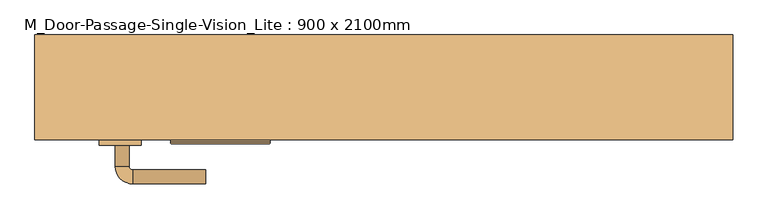
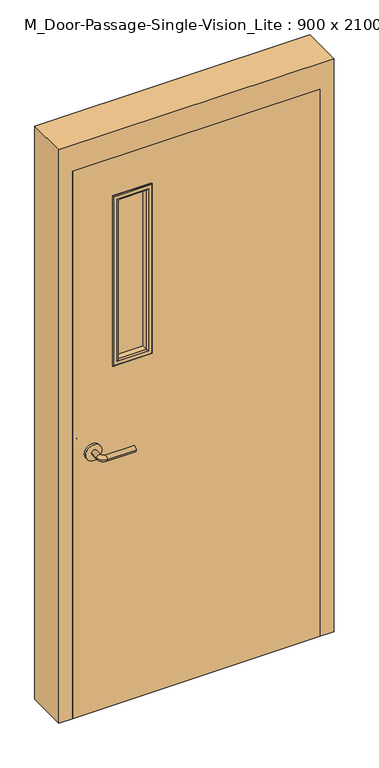
"""IFC4 building model written with IfcOpenShell, lengths in millimetres: door geometry, M_Door-Passage-Single-Vision_Lite : 900 x 2100mm."""

import ifcopenshell
import ifcopenshell.guid

model = None  # the IFC model being written
_history = None  # IfcOwnerHistory: only IFC2X3 demands one
_inside = {}  # id of a spatial element -> (the spatial element, [elements in it])
_under = {}  # id of a project, library or spatial element -> (it, [spatial elements below it])
_declared = {}  # id of a project -> (the project, [libraries it declares])
_typed = {}  # id of a type object -> (the type object, [elements of that type])
_made_of = {}  # id of a material, layer set ... -> (it, [elements and type objects made of it])


def new_model(schema):
    """Start an empty IFC model of exactly this schema.

    Asked for "IFC4X3", IfcOpenShell would pick the latest addendum, in which some entities
    have other attributes; the version numbers below select the first issue.
    IFC2X3 requires an IfcOwnerHistory on every rooted entity: one is made here for all.
    """
    global model, _history
    if schema == "IFC4X3":
        model = ifcopenshell.file(schema_version=(4, 3, 0, 0))
    else:
        model = ifcopenshell.file(schema=schema)
    _inside.clear()
    _under.clear()
    _declared.clear()
    _typed.clear()
    _made_of.clear()
    _history = None
    if model.schema == "IFC2X3":
        org = make("IfcOrganization", Name="unknown")
        user = make(
            "IfcPersonAndOrganization",
            ThePerson=make("IfcPerson", FamilyName="unknown"),
            TheOrganization=org,
        )
        app = make(
            "IfcApplication",
            ApplicationDeveloper=org,
            Version="unknown",
            ApplicationFullName="unknown",
            ApplicationIdentifier="unknown",
        )
        _history = make(
            "IfcOwnerHistory",
            OwningUser=user,
            OwningApplication=app,
            ChangeAction="ADDED",
            CreationDate=0,
        )
    return model


def make(cls, **values):
    """One entity of the class cls with the attributes given. An attribute that is None is left unset."""
    return model.create_entity(
        cls, **{name: value for name, value in values.items() if value is not None}
    )


def rooted(cls, **values):
    """An entity with a GlobalId (a new one), such as an element, a storey or a relation."""
    return make(cls, GlobalId=ifcopenshell.guid.new(), OwnerHistory=_history, **values)


def si_unit(unit_type, name, prefix=None):
    """IfcSIUnit, for example si_unit("LENGTHUNIT", "METRE", prefix="MILLI")."""
    return make("IfcSIUnit", UnitType=unit_type, Prefix=prefix, Name=name)


def assignment(units):
    """IfcUnitAssignment: the units of a project."""
    return None if units is None else make("IfcUnitAssignment", Units=units)


def point(xyz):
    """IfcCartesianPoint."""
    return None if xyz is None else make("IfcCartesianPoint", Coordinates=xyz)


def direction(xyz):
    """IfcDirection."""
    return None if xyz is None else make("IfcDirection", DirectionRatios=xyz)


def frame(location, z_axis=None, x_axis=None):
    """IfcAxis2Placement3D, a coordinate frame: its origin and axes. An axis left out is left unset."""
    return make(
        "IfcAxis2Placement3D",
        Location=point(location),
        Axis=direction(z_axis),
        RefDirection=direction(x_axis),
    )


def frame_2d(location, x_axis=None):
    """IfcAxis2Placement2D, a coordinate frame in the plane: its origin and x axis."""
    return make(
        "IfcAxis2Placement2D", Location=point(location), RefDirection=direction(x_axis)
    )


def origin():
    """The frame at (0, 0, 0) with its axes left unset."""
    return frame((0.0, 0.0, 0.0))


def place(relative_to, where):
    """IfcLocalPlacement: puts the frame where relative to a parent placement (None: the world)."""
    return make(
        "IfcLocalPlacement", PlacementRelTo=relative_to, RelativePlacement=where
    )


def context(
    kind, dimensions, precision=None, world=None, true_north=None, identifier=None
):
    """IfcGeometricRepresentationContext, for example the 3D "Model" context."""
    return make(
        "IfcGeometricRepresentationContext",
        ContextIdentifier=identifier,
        ContextType=kind,
        CoordinateSpaceDimension=dimensions,
        Precision=precision,
        WorldCoordinateSystem=world,
        TrueNorth=true_north,
    )


def project(units=None, contexts=None):
    """IfcProject with its units and contexts."""
    return rooted(
        "IfcProject",
        Name="project",
        RepresentationContexts=contexts,
        UnitsInContext=assignment(units),
    )


def spatial(cls, under=None, at=None, **own):
    """A site, building, storey or space (cls), placed at a placement, below another one or the project."""
    s = rooted(cls, ObjectPlacement=at, **own)
    if under is not None:
        _under.setdefault(under.id(), (under, []))[1].append(s)
    return s


def polyline(points):
    """IfcPolyline through the points."""
    return make("IfcPolyline", Points=[point(p) for p in points])


def circle_curve(where, radius):
    """IfcCircle in the frame where."""
    return make("IfcCircle", Position=where, Radius=radius)


def ellipse_curve(where, semi_axis1, semi_axis2):
    """IfcEllipse in the frame where."""
    return make(
        "IfcEllipse", Position=where, SemiAxis1=semi_axis1, SemiAxis2=semi_axis2
    )


def trimmed(basis, trim1, trim2, sense, master):
    """IfcTrimmedCurve: the piece of a basis curve between two trims."""
    return make(
        "IfcTrimmedCurve",
        BasisCurve=basis,
        Trim1=trim1,
        Trim2=trim2,
        SenseAgreement=sense,
        MasterRepresentation=master,
    )


def segment(curve, same_sense, transition):
    """IfcCompositeCurveSegment."""
    return make(
        "IfcCompositeCurveSegment",
        Transition=transition,
        SameSense=same_sense,
        ParentCurve=curve,
    )


def composite_curve(segments, self_intersect=None):
    """IfcCompositeCurve: segments joined end to end."""
    return make("IfcCompositeCurve", Segments=segments, SelfIntersect=self_intersect)


def outline(outer, holes=None, kind="AREA"):
    """IfcArbitraryClosedProfileDef: a profile drawn as a closed curve; with holes, ...WithVoids."""
    if holes is None:
        return make("IfcArbitraryClosedProfileDef", ProfileType=kind, OuterCurve=outer)
    return make(
        "IfcArbitraryProfileDefWithVoids",
        ProfileType=kind,
        OuterCurve=outer,
        InnerCurves=holes,
    )


def extrude(swept, where, along, depth):
    """IfcExtrudedAreaSolid: the profile swept, set in the frame where, extruded along a direction by depth."""
    return make(
        "IfcExtrudedAreaSolid",
        SweptArea=swept,
        Position=where,
        ExtrudedDirection=direction(along),
        Depth=depth,
    )


def faces_of(points, faces, orient=None, outer=None):
    """IfcFace entities. A face is a list of loops; a loop is a list of indices into points, from 0.

    orient and outer hold one flag for each loop. By default every Orientation is true, the
    first loop of a face is its IfcFaceOuterBound and the others are IfcFaceBound.
    """
    made = []
    for i, loops in enumerate(faces):
        bounds = []
        for j, loop in enumerate(loops):
            is_outer = j == 0 if outer is None else outer[i][j]
            bounds.append(
                make(
                    "IfcFaceOuterBound" if is_outer else "IfcFaceBound",
                    Bound=make("IfcPolyLoop", Polygon=[points[k] for k in loop]),
                    Orientation=True if orient is None else orient[i][j],
                )
            )
        made.append(make("IfcFace", Bounds=bounds))
    return made


def faceted_brep(points, faces, orient=None, outer=None, voids=None):
    """IfcFacetedBrep: a solid bounded by flat faces; with voids (closed shells), ...WithVoids."""
    shared = [point(p) for p in points]
    hull = make("IfcClosedShell", CfsFaces=faces_of(shared, faces, orient, outer))
    if voids is None:
        return make("IfcFacetedBrep", Outer=hull)
    return make(
        "IfcFacetedBrepWithVoids",
        Outer=hull,
        Voids=[
            make(cls, CfsFaces=faces_of(shared, fs, o, b)) for cls, fs, o, b in voids
        ],
    )


def shape(context_of_items, identifier, shape_type, items):
    """IfcShapeRepresentation: the items that make up one representation, for example the "Body"."""
    return make(
        "IfcShapeRepresentation",
        ContextOfItems=context_of_items,
        RepresentationIdentifier=identifier,
        RepresentationType=shape_type,
        Items=items,
    )


def source(mapping_origin, context_of_items, identifier, shape_type, items):
    """IfcRepresentationMap: a shape defined once, which mapped items show again and again."""
    return make(
        "IfcRepresentationMap",
        MappingOrigin=mapping_origin,
        MappedRepresentation=shape(context_of_items, identifier, shape_type, items),
    )


def transform(
    local_origin,
    x_axis=None,
    y_axis=None,
    z_axis=None,
    scale=None,
    scale2=None,
    scale3=None,
    uniform=True,
):
    """IfcCartesianTransformationOperator3D, or its non-uniform kind. x_axis, y_axis, z_axis: its Axis1, 2, 3."""
    if uniform:
        return make(
            "IfcCartesianTransformationOperator3D",
            Axis1=direction(x_axis),
            Axis2=direction(y_axis),
            LocalOrigin=point(local_origin),
            Scale=scale,
            Axis3=direction(z_axis),
        )
    return make(
        "IfcCartesianTransformationOperator3DnonUniform",
        Axis1=direction(x_axis),
        Axis2=direction(y_axis),
        LocalOrigin=point(local_origin),
        Scale=scale,
        Axis3=direction(z_axis),
        Scale2=scale2,
        Scale3=scale3,
    )


def mapped(mapping_source, mapping_target):
    """IfcMappedItem: shows the shape of a source again, moved by a transform."""
    return make(
        "IfcMappedItem", MappingSource=mapping_source, MappingTarget=mapping_target
    )


def made_of(thing, what):
    """Note that an element or type object is made of a material, layer set ...; save() writes the relation."""
    if what is not None:
        _made_of.setdefault(what.id(), (what, []))[1].append(thing)
    return thing


def element(
    cls,
    number,
    at=None,
    inside=None,
    cuts=None,
    type_object=None,
    material=None,
    context=None,
    identifier="Body",
    shape_type=None,
    held_by="IfcProductDefinitionShape",
    body=None,
    shapes=None,
    **own,
):
    """One element of the class cls, such as IfcWall. Its Tag is "e" and its number.

    at: its placement. inside: the storey or other place that contains it. cuts: it is an
    opening in that element (IfcRelVoidsElement). A single representation is given by context,
    identifier, shape_type and body (its items); several are given by shapes. held_by: the class
    of the entity that holds the representations. save() writes the other relations.
    """
    e = rooted(cls, Tag="e%d" % number, ObjectPlacement=at, **own)
    if body is not None:
        shapes = [shape(context, identifier, shape_type, body)]
    if shapes is not None:
        e.Representation = make(held_by, Representations=shapes)
    if inside is not None:
        _inside.setdefault(inside.id(), (inside, []))[1].append(e)
    if cuts is not None:
        rooted(
            "IfcRelVoidsElement", RelatingBuildingElement=cuts, RelatedOpeningElement=e
        )
    if type_object is not None:
        _typed.setdefault(type_object.id(), (type_object, []))[1].append(e)
    return made_of(e, material)


def aggregate(whole, parts):
    """IfcRelAggregates: a whole, such as a stair, and the parts it consists of."""
    return rooted("IfcRelAggregates", RelatingObject=whole, RelatedObjects=parts)


def save(model, path):
    """Write the relations noted so far, then the file.

    IfcRelAggregates (storeys below a building ...), IfcRelContainedInSpatialStructure (elements
    in a storey), IfcRelDefinesByType, IfcRelAssociatesMaterial and IfcRelDeclares: one each for
    every whole, place, type object, material and project.
    """
    for whole, parts in _under.values():
        aggregate(whole, parts)
    for where, things in _inside.values():
        rooted(
            "IfcRelContainedInSpatialStructure",
            RelatedElements=things,
            RelatingStructure=where,
        )
    for kind, things in _typed.values():
        rooted("IfcRelDefinesByType", RelatedObjects=things, RelatingType=kind)
    for what, things in _made_of.values():
        rooted("IfcRelAssociatesMaterial", RelatedObjects=things, RelatingMaterial=what)
    for by, libraries in _declared.values():
        rooted("IfcRelDeclares", RelatingContext=by, RelatedDefinitions=libraries)
    model.write(path)


def plane_surface(at):
    """IfcPlane: the flat surface through the origin of the frame at, square to its z axis."""
    return make("IfcPlane", Position=at)


def cylinder_surface(at, radius):
    """IfcCylindricalSurface: all points at the distance radius from the z axis of the frame at."""
    return make("IfcCylindricalSurface", Position=at, Radius=radius)


def revolved_surface(curve, axis_point, axis_direction):
    """IfcSurfaceOfRevolution: the curve turned about the line through axis_point along axis_direction."""
    return make(
        "IfcSurfaceOfRevolution",
        SweptCurve=make("IfcArbitraryOpenProfileDef", ProfileType="CURVE", Curve=curve),
        AxisPosition=make("IfcAxis1Placement", Location=point(axis_point), Axis=direction(axis_direction)),
    )


def advanced_brep(points, edges, surfaces, faces):
    """IfcAdvancedBrep: a solid bounded by faces that lie on surfaces and meet in shared edges.

    An edge is (start, end): straight between two places in points (the first is 0);
    or (start, end, curve); or (start, end, curve, False) where it runs against its curve.
    A face is (place in surfaces, loops), or (place, loops, False) where it looks against
    its surface's normal. A loop lists edges by number (the first is 1), with a minus sign
    where the edge is run from its end to its start. The first loop is the outer one.
    """
    corners = [point(p) for p in points]
    vertices = [make("IfcVertexPoint", VertexGeometry=c) for c in corners]
    made = []
    for start, end, *more in edges:
        made.append(
            make(
                "IfcEdgeCurve",
                EdgeStart=vertices[start],
                EdgeEnd=vertices[end],
                EdgeGeometry=more[0] if more else make("IfcPolyline", Points=[corners[start], corners[end]]),
                SameSense=more[1] if len(more) > 1 else True,
            )
        )
    hull = []
    for where, loops, *sense in faces:
        bounds = []
        for j, loop in enumerate(loops):
            ring = [make("IfcOrientedEdge", EdgeElement=made[abs(k) - 1], Orientation=k > 0) for k in loop]
            bounds.append(
                make(
                    "IfcFaceOuterBound" if j == 0 else "IfcFaceBound",
                    Bound=make("IfcEdgeLoop", EdgeList=ring),
                    Orientation=True,
                )
            )
        hull.append(make("IfcAdvancedFace", Bounds=bounds, FaceSurface=surfaces[where], SameSense=sense[0] if sense else True))
    return make("IfcAdvancedBrep", Outer=make("IfcClosedShell", CfsFaces=hull))


def m_door_passage_single_vision_lite_900_x_2100mm_db62f7dd(model_context):
    return source(origin(), model_context, "Body", "SolidModel", [
        advanced_brep(
        [(-384.990625, 9.15, 1000.0), (-364.990625, 9.15, 1000.0), (-384.990625, 39.15, 1000.0), (-364.990625, 39.15, 1000.0), (-359.990625, 44.15, 1000.0), (-359.990625, 64.15, 1000.0), (-254.990625, 64.15, 1000.0), (-254.990625, 44.15, 1000.0)],
        [
            (0, 1, circle_curve(frame((-374.990625, 9.15, 1000.0), z_axis=(0.0, -1.0, 0.0), x_axis=(1.0, 0.0, 0.0)), 10.0)),
            (1, 0, circle_curve(frame((-374.990625, 9.15, 1000.0), z_axis=(0.0, -1.0, 0.0), x_axis=(1.0, 0.0, 0.0)), 10.0)),
            (0, 2),
            (2, 3, circle_curve(frame((-374.990625, 39.15, 1000.0), z_axis=(0.0, -1.0, 0.0), x_axis=(1.0, 0.0, 0.0)), 10.0)),
            (3, 1),
            (3, 2, circle_curve(frame((-374.990625, 39.15, 1000.0), z_axis=(0.0, -1.0, 0.0), x_axis=(1.0, 0.0, 0.0)), 10.0)),
            (4, 3, circle_curve(frame((-359.990625, 39.15, 1000.0), z_axis=(0.0, 0.0, 1.0), x_axis=(-1.0, 0.0, 0.0)), 5.0)),
            (2, 5, circle_curve(frame((-359.990625, 39.15, 1000.0), z_axis=(0.0, 0.0, -1.0), x_axis=(-1.0, 0.0, 0.0)), 25.0)),
            (5, 4, circle_curve(frame((-359.990625, 54.15, 1000.0), z_axis=(-1.0, 0.0, 0.0), x_axis=(0.0, -1.0, 0.0)), 10.0)),
            (4, 5, circle_curve(frame((-359.990625, 54.15, 1000.0), z_axis=(-1.0, 0.0, 0.0), x_axis=(0.0, -1.0, 0.0)), 10.0)),
            (6, 7, circle_curve(frame((-254.990625, 54.15, 1000.0), z_axis=(1.0, 0.0, 0.0), x_axis=(0.0, -1.0, 0.0)), 10.0)),
            (7, 6, circle_curve(frame((-254.990625, 54.15, 1000.0), z_axis=(1.0, 0.0, 0.0), x_axis=(0.0, -1.0, 0.0)), 10.0)),
            (5, 6),
            (7, 4),
        ],
        [
            plane_surface(frame((-374.990625, 9.15, 1000.0), z_axis=(0.0, -1.0, 0.0), x_axis=(0.0, 0.0, 1.0))),
            cylinder_surface(frame((-374.990625, 9.15, 1000.0), z_axis=(0.0, -1.0, 0.0), x_axis=(1.0, 0.0, 0.0)), 10.0),
            revolved_surface(trimmed(ellipse_curve(frame((-374.990625, 39.15, 1000.0), z_axis=(0.0, -1.0, 0.0), x_axis=(1.0, 0.0, 0.0)), 10.0, 10.0), [point((-384.990625, 39.15, 1000.0))], [point((-364.990625, 39.15, 1000.0))], True, "CARTESIAN"), (-359.990625, 39.15, 1000.0), (0.0, 0.0, -1.0)),
            revolved_surface(trimmed(ellipse_curve(frame((-374.990625, 39.15, 1000.0), z_axis=(0.0, -1.0, 0.0), x_axis=(1.0, 0.0, 0.0)), 10.0, 10.0), [point((-364.990625, 39.15, 1000.0))], [point((-384.990625, 39.15, 1000.0))], True, "CARTESIAN"), (-359.990625, 39.15, 1000.0), (0.0, 0.0, -1.0)),
            plane_surface(frame((-254.990625, 54.15, 1000.0), z_axis=(1.0, 0.0, 0.0), x_axis=(0.0, 0.0, 1.0))),
            cylinder_surface(frame((-359.990625, 54.15, 1000.0), z_axis=(-1.0, 0.0, 0.0), x_axis=(0.0, -1.0, 0.0)), 10.0),
        ],
        [
            (0, [[1, 2]]),
            (1, [[-1, 3, 4, 5]]),
            (1, [[-2, -5, 6, -3]]),
            (2, [[7, -4, 8, 9]]),
            (3, [[-8, -6, -7, 10]]),
            (4, [[11, 12]]),
            (5, [[-9, 13, -12, 14]]),
            (5, [[-10, -14, -11, -13]]),
        ],
    ),
        extrude(outline(composite_curve([segment(trimmed(circle_curve(frame_2d((1000.0, -377.490625)), 30.0), [point((1000.0, -407.490625))], [point((1000.0, -347.490625))], False, "CARTESIAN"), True, "CONTINUOUS"), segment(trimmed(circle_curve(frame_2d((1000.0, -377.490625)), 30.0), [point((1000.0, -347.490625))], [point((1000.0, -407.490625))], False, "CARTESIAN"), True, "CONTINUOUS")], self_intersect=False)), frame((0.0, 1.15, 0.0), z_axis=(0.0, 1.0, 0.0), x_axis=(0.0, 0.0, 1.0)), (0.0, 0.0, 1.0), 8.0),
        advanced_brep(
        [(-384.990625, -51.85, 1000.0), (-364.990625, -51.85, 1000.0), (-364.990625, -81.85, 1000.0), (-384.990625, -81.85, 1000.0), (-359.990625, -86.85, 1000.0), (-359.990625, -106.85, 1000.0), (-254.990625, -106.85, 1000.0), (-254.990625, -86.85, 1000.0)],
        [
            (0, 1, circle_curve(frame((-374.990625, -51.85, 1000.0), z_axis=(0.0, 1.0, 0.0), x_axis=(1.0, 0.0, 0.0)), 10.0)),
            (1, 0, circle_curve(frame((-374.990625, -51.85, 1000.0), z_axis=(0.0, 1.0, 0.0), x_axis=(1.0, 0.0, 0.0)), 10.0)),
            (1, 2),
            (2, 3, circle_curve(frame((-374.990625, -81.85, 1000.0), z_axis=(0.0, 1.0, 0.0), x_axis=(1.0, 0.0, 0.0)), 10.0)),
            (3, 0),
            (3, 2, circle_curve(frame((-374.990625, -81.85, 1000.0), z_axis=(0.0, 1.0, 0.0), x_axis=(1.0, 0.0, 0.0)), 10.0)),
            (4, 5, circle_curve(frame((-359.990625, -96.85, 1000.0), z_axis=(-1.0, 0.0, 0.0), x_axis=(0.0, 1.0, 0.0)), 10.0)),
            (5, 3, circle_curve(frame((-359.990625, -81.85, 1000.0), z_axis=(0.0, 0.0, -1.0), x_axis=(-1.0, 0.0, 0.0)), 25.0)),
            (2, 4, circle_curve(frame((-359.990625, -81.85, 1000.0), z_axis=(0.0, 0.0, 1.0), x_axis=(-1.0, 0.0, 0.0)), 5.0)),
            (5, 4, circle_curve(frame((-359.990625, -96.85, 1000.0), z_axis=(-1.0, 0.0, 0.0), x_axis=(0.0, 1.0, 0.0)), 10.0)),
            (6, 7, circle_curve(frame((-254.990625, -96.85, 1000.0), z_axis=(1.0, 0.0, 0.0), x_axis=(0.0, 1.0, 0.0)), 10.0)),
            (7, 6, circle_curve(frame((-254.990625, -96.85, 1000.0), z_axis=(1.0, 0.0, 0.0), x_axis=(0.0, 1.0, 0.0)), 10.0)),
            (4, 7),
            (6, 5),
        ],
        [
            plane_surface(frame((-374.990625, -51.85, 1000.0), z_axis=(0.0, 1.0, 0.0), x_axis=(0.0, 0.0, 1.0))),
            cylinder_surface(frame((-374.990625, -51.85, 1000.0), z_axis=(0.0, 1.0, 0.0), x_axis=(1.0, 0.0, 0.0)), 10.0),
            revolved_surface(trimmed(ellipse_curve(frame((-374.990625, -81.85, 1000.0), z_axis=(0.0, -1.0, 0.0), x_axis=(1.0, 0.0, 0.0)), 10.0, 10.0), [point((-384.990625, -81.85, 1000.0))], [point((-364.990625, -81.85, 1000.0))], True, "CARTESIAN"), (-359.990625, -81.85, 1000.0), (0.0, 0.0, -1.0)),
            revolved_surface(trimmed(ellipse_curve(frame((-374.990625, -81.85, 1000.0), z_axis=(0.0, -1.0, 0.0), x_axis=(1.0, 0.0, 0.0)), 10.0, 10.0), [point((-364.990625, -81.85, 1000.0))], [point((-384.990625, -81.85, 1000.0))], True, "CARTESIAN"), (-359.990625, -81.85, 1000.0), (0.0, 0.0, -1.0)),
            plane_surface(frame((-254.990625, -96.85, 1000.0), z_axis=(1.0, 0.0, 0.0), x_axis=(0.0, 0.0, 1.0))),
            cylinder_surface(frame((-359.990625, -96.85, 1000.0), z_axis=(-1.0, 0.0, 0.0), x_axis=(0.0, 1.0, 0.0)), 10.0),
        ],
        [
            (0, [[1, 2]]),
            (1, [[3, 4, 5, -2]]),
            (1, [[-5, 6, -3, -1]]),
            (2, [[7, 8, -4, 9]]),
            (3, [[10, -9, -6, -8]]),
            (4, [[11, 12]]),
            (5, [[13, -11, 14, -7]]),
            (5, [[-14, -12, -13, -10]]),
        ],
    ),
        extrude(outline(composite_curve([segment(trimmed(circle_curve(frame_2d((1000.0, -377.490625)), 30.0), [point((1000.0, -407.490625))], [point((1000.0, -347.490625))], False, "CARTESIAN"), True, "CONTINUOUS"), segment(trimmed(circle_curve(frame_2d((1000.0, -377.490625)), 30.0), [point((1000.0, -347.490625))], [point((1000.0, -407.490625))], False, "CARTESIAN"), True, "CONTINUOUS")], self_intersect=False)), frame((0.0, -51.85, 0.0), z_axis=(0.0, 1.0, 0.0), x_axis=(0.0, 0.0, 1.0)), (0.0, 0.0, 1.0), 8.0),
        extrude(outline(polyline([(2100.0, -450.0), (0.0, -450.0), (0.0, 450.0), (2100.0, 450.0), (2100.0, -450.0)]), holes=[polyline([(1947.6, -297.6), (1947.6, -170.6), (1312.6, -170.6), (1312.6, -297.6), (1947.6, -297.6)])]), frame((0.0, -43.85, 0.0), z_axis=(0.0, 1.0, 0.0), x_axis=(0.0, 0.0, 1.0)), (0.0, 0.0, 1.0), 45.0),
        faceted_brep([(450.0, 5.9125, 0.0), (434.125, 5.9125, 0.0), (434.125, 56.9375, 0.0), (450.0, 56.9375, 0.0), (450.0, 106.15, 0.0), (500.0, 106.15, 0.0), (500.0, -43.85, 0.0), (450.0, -43.85, 0.0), (450.0, -43.85, 2100.0), (450.0, 5.9125, 2100.0), (500.0, -43.85, 2200.0), (-500.0, -43.85, 2200.0), (-500.0, -43.85, 0.0), (-450.0, -43.85, 0.0), (-450.0, -43.85, 2100.0), (500.0, 106.15, 2200.0), (450.0, 106.15, 2100.0), (-450.0, 106.15, 2100.0), (-450.0, 106.15, 0.0), (-500.0, 106.15, 0.0), (-500.0, 106.15, 2200.0), (450.0, 56.9375, 2100.0), (434.125, 56.9375, 2084.125), (-434.125, 56.9375, 2084.125), (-434.125, 56.9375, 0.0), (-450.0, 56.9375, 0.0), (-450.0, 56.9375, 2100.0), (434.125, 5.9125, 2084.125), (-450.0, 5.9125, 2100.0), (-450.0, 5.9125, 0.0), (-434.125, 5.9125, 0.0), (-434.125, 5.9125, 2084.125)], [[[0, 1, 2, 3, 4, 5, 6, 7]], [[7, 8, 9, 0]], [[6, 10, 11, 12, 13, 14, 8, 7]], [[5, 15, 10, 6]], [[4, 16, 17, 18, 19, 20, 15, 5]], [[3, 21, 16, 4]], [[2, 22, 23, 24, 25, 26, 21, 3]], [[1, 27, 22, 2]], [[0, 9, 28, 29, 30, 31, 27, 1]], [[8, 14, 28, 9]], [[16, 21, 26, 17]], [[22, 27, 31, 23]], [[12, 19, 18, 25, 24, 30, 29, 13]], [[13, 29, 28, 14]], [[11, 20, 19, 12]], [[17, 26, 25, 18]], [[23, 31, 30, 24]], [[15, 20, 11, 10]]]),
        extrude(outline(polyline([(-170.6, -18.85), (-170.6, -23.85), (-297.6, -23.85), (-297.6, -18.85), (-170.6, -18.85)])), frame((0.0, 0.0, 1312.6), z_axis=(0.0, 0.0, 1.0), x_axis=(1.0, 0.0, 0.0)), (0.0, 0.0, 1.0), 635.0),
        advanced_brep(
        [(-297.6, -23.85, 1947.6), (-297.6, -23.85, 1312.6), (-297.6, -43.85, 1312.6), (-297.6, -43.85, 1947.6), (-285.6, -44.85, 1935.6), (-285.6, -44.85, 1324.6), (-285.6, -23.85, 1324.6), (-285.6, -23.85, 1935.6), (-290.6, -49.85, 1940.6), (-290.6, -49.85, 1319.6), (-305.6, -47.85, 1955.6), (-305.6, -47.85, 1304.6), (-303.6, -49.85, 1306.6), (-303.6, -49.85, 1953.6), (-305.6, -43.85, 1955.6), (-305.6, -43.85, 1304.6), (-170.6, -23.85, 1312.6), (-170.6, -43.85, 1312.6), (-182.6, -44.85, 1324.6), (-182.6, -23.85, 1324.6), (-177.6, -49.85, 1319.6), (-162.6, -47.85, 1304.6), (-164.6, -49.85, 1306.6), (-162.6, -43.85, 1304.6), (-170.6, -23.85, 1947.6), (-170.6, -43.85, 1947.6), (-182.6, -44.85, 1935.6), (-182.6, -23.85, 1935.6), (-177.6, -49.85, 1940.6), (-162.6, -47.85, 1955.6), (-164.6, -49.85, 1953.6), (-162.6, -43.85, 1955.6)],
        [
            (0, 1),
            (1, 2),
            (2, 3),
            (3, 0),
            (4, 5),
            (5, 6),
            (6, 7),
            (7, 4),
            (8, 9),
            (9, 5, ellipse_curve(frame((-290.6, -44.85, 1319.6), z_axis=(-0.7071067811865475, 0.0, 0.7071067811865475), x_axis=(0.7071067811865474, 0.0, 0.7071067811865476)), 7.0710678, 5.0)),
            (4, 8, ellipse_curve(frame((-290.6, -44.85, 1940.6), z_axis=(-0.7071067811865475, 0.0, -0.7071067811865475), x_axis=(-0.7071067811865474, 0.0, 0.7071067811865476)), 7.0710678, 5.0)),
            (10, 11),
            (11, 12, ellipse_curve(frame((-303.6, -47.85, 1306.6), z_axis=(-0.7071067811865475, 0.0, 0.7071067811865475), x_axis=(0.7071067811865474, 0.0, 0.7071067811865476)), 2.8284271, 2.0)),
            (12, 13),
            (13, 10, ellipse_curve(frame((-303.6, -47.85, 1953.6), z_axis=(-0.7071067811865475, 0.0, -0.7071067811865475), x_axis=(-0.7071067811865474, 0.0, 0.7071067811865476)), 2.8284271, 2.0)),
            (14, 15),
            (15, 11),
            (10, 14),
            (1, 16),
            (16, 17),
            (17, 2),
            (5, 18),
            (18, 19),
            (19, 6),
            (9, 20),
            (20, 18, ellipse_curve(frame((-177.6, -44.85, 1319.6), z_axis=(-0.7071067811865475, 0.0, -0.7071067811865475), x_axis=(-0.7071067811865476, 0.0, 0.7071067811865474)), 7.0710678, 5.0)),
            (11, 21),
            (21, 22, ellipse_curve(frame((-164.6, -47.85, 1306.6), z_axis=(-0.7071067811865475, 0.0, -0.7071067811865475), x_axis=(-0.7071067811865476, 0.0, 0.7071067811865474)), 2.8284271, 2.0)),
            (22, 12),
            (15, 23),
            (23, 21),
            (16, 24),
            (24, 25),
            (25, 17),
            (18, 26),
            (26, 27),
            (27, 19),
            (20, 28),
            (28, 26, ellipse_curve(frame((-177.6, -44.85, 1940.6), z_axis=(0.7071067811865475, 0.0, -0.7071067811865475), x_axis=(-0.7071067811865474, 0.0, -0.7071067811865476)), 7.0710678, 5.0)),
            (21, 29),
            (29, 30, ellipse_curve(frame((-164.6, -47.85, 1953.6), z_axis=(0.7071067811865475, 0.0, -0.7071067811865475), x_axis=(-0.7071067811865474, 0.0, -0.7071067811865476)), 2.8284271, 2.0)),
            (30, 22),
            (23, 31),
            (31, 29),
            (14, 31),
            (25, 3),
            (24, 0),
            (27, 7),
            (26, 4),
            (28, 8),
            (30, 13),
            (29, 10),
        ],
        [
            plane_surface(frame((-297.6, -43.85, 1947.6), z_axis=(-1.0, 0.0, 0.0), x_axis=(0.0, 0.0, -1.0))),
            plane_surface(frame((-285.6, -23.85, 1935.6), z_axis=(1.0, 0.0, 0.0), x_axis=(0.0, 0.0, -1.0))),
            cylinder_surface(frame((-290.6, -44.85, 1947.6), z_axis=(0.0, 0.0, 1.0), x_axis=(-1.0, 0.0, 0.0)), 5.0),
            cylinder_surface(frame((-303.6, -47.85, 1947.6), z_axis=(0.0, 0.0, 1.0), x_axis=(-1.0, 0.0, 0.0)), 2.0),
            plane_surface(frame((-305.6, -47.85, 1955.6), z_axis=(-1.0, 0.0, 0.0), x_axis=(0.0, 0.0, -1.0))),
            plane_surface(frame((-297.6, -43.85, 1312.6), z_axis=(0.0, 0.0, -1.0), x_axis=(1.0, 0.0, 0.0))),
            plane_surface(frame((-285.6, -23.85, 1324.6), z_axis=(0.0, 0.0, 1.0), x_axis=(1.0, 0.0, 0.0))),
            cylinder_surface(frame((-297.6, -44.85, 1319.6), z_axis=(-1.0, 0.0, 0.0), x_axis=(0.0, 0.0, -1.0)), 5.0),
            cylinder_surface(frame((-297.6, -47.85, 1306.6), z_axis=(-1.0, 0.0, 0.0), x_axis=(0.0, 0.0, -1.0)), 2.0),
            plane_surface(frame((-305.6, -47.85, 1304.6), z_axis=(0.0, 0.0, -1.0), x_axis=(1.0, 0.0, 0.0))),
            plane_surface(frame((-170.6, -43.85, 1312.6), z_axis=(1.0, 0.0, 0.0), x_axis=(0.0, 0.0, 1.0))),
            plane_surface(frame((-182.6, -23.85, 1324.6), z_axis=(-1.0, 0.0, 0.0), x_axis=(0.0, 0.0, 1.0))),
            cylinder_surface(frame((-177.6, -44.85, 1312.6), z_axis=(0.0, 0.0, -1.0), x_axis=(1.0, 0.0, 0.0)), 5.0),
            cylinder_surface(frame((-164.6, -47.85, 1312.6), z_axis=(0.0, 0.0, -1.0), x_axis=(1.0, 0.0, 0.0)), 2.0),
            plane_surface(frame((-162.6, -47.85, 1304.6), z_axis=(1.0, 0.0, 0.0), x_axis=(0.0, 0.0, 1.0))),
            plane_surface(frame((-162.6, -43.85, 1955.6), z_axis=(0.0, 1.0, 0.0), x_axis=(-1.0, 0.0, 0.0))),
            plane_surface(frame((-170.6, -43.85, 1947.6), z_axis=(0.0, 0.0, 1.0), x_axis=(-1.0, 0.0, 0.0))),
            plane_surface(frame((-170.6, -23.85, 1947.6), z_axis=(0.0, 1.0, 0.0), x_axis=(-1.0, 0.0, 0.0))),
            plane_surface(frame((-182.6, -23.85, 1935.6), z_axis=(0.0, 0.0, -1.0), x_axis=(-1.0, 0.0, 0.0))),
            cylinder_surface(frame((-170.6, -44.85, 1940.6), z_axis=(1.0, 0.0, 0.0), x_axis=(0.0, 0.0, 1.0)), 5.0),
            plane_surface(frame((-177.6, -49.85, 1940.6), z_axis=(0.0, -1.0, 0.0), x_axis=(-1.0, 0.0, 0.0))),
            cylinder_surface(frame((-170.6, -47.85, 1953.6), z_axis=(1.0, 0.0, 0.0), x_axis=(0.0, 0.0, 1.0)), 2.0),
            plane_surface(frame((-162.6, -47.85, 1955.6), z_axis=(0.0, 0.0, 1.0), x_axis=(-1.0, 0.0, 0.0))),
        ],
        [
            (0, [[1, 2, 3, 4]]),
            (1, [[5, 6, 7, 8]]),
            (2, [[9, 10, -5, 11]]),
            (3, [[12, 13, 14, 15]]),
            (4, [[16, 17, -12, 18]]),
            (5, [[19, 20, 21, -2]]),
            (6, [[22, 23, 24, -6]]),
            (7, [[25, 26, -22, -10]]),
            (8, [[27, 28, 29, -13]]),
            (9, [[30, 31, -27, -17]]),
            (10, [[32, 33, 34, -20]]),
            (11, [[35, 36, 37, -23]]),
            (12, [[38, 39, -35, -26]]),
            (13, [[40, 41, 42, -28]]),
            (14, [[43, 44, -40, -31]]),
            (15, [[-16, 45, -43, -30], [-3, -21, -34, 46]]),
            (16, [[47, -4, -46, -33]]),
            (17, [[-1, -47, -32, -19], [-7, -24, -37, 48]]),
            (18, [[49, -8, -48, -36]]),
            (19, [[50, -11, -49, -39]]),
            (20, [[-14, -29, -42, 51], [-9, -50, -38, -25]]),
            (21, [[52, -15, -51, -41]]),
            (22, [[-45, -18, -52, -44]]),
        ],
    ),
        advanced_brep(
        [(-297.6, -18.85, 1312.6), (-297.6, -18.85, 1947.6), (-297.6, 1.15, 1947.6), (-297.6, 1.15, 1312.6), (-285.6, 2.15, 1324.6), (-285.6, 2.15, 1935.6), (-285.6, -18.85, 1935.6), (-285.6, -18.85, 1324.6), (-290.6, 7.15, 1319.6), (-290.6, 7.15, 1940.6), (-305.6, 5.15, 1304.6), (-305.6, 5.15, 1955.6), (-303.6, 7.15, 1953.6), (-303.6, 7.15, 1306.6), (-305.6, 1.15, 1304.6), (-305.6, 1.15, 1955.6), (-170.6, -18.85, 1947.6), (-170.6, 1.15, 1947.6), (-182.6, 2.15, 1935.6), (-182.6, -18.85, 1935.6), (-177.6, 7.15, 1940.6), (-162.6, 5.15, 1955.6), (-164.6, 7.15, 1953.6), (-162.6, 1.15, 1955.6), (-170.6, -18.85, 1312.6), (-170.6, 1.15, 1312.6), (-182.6, 2.15, 1324.6), (-182.6, -18.85, 1324.6), (-177.6, 7.15, 1319.6), (-162.6, 5.15, 1304.6), (-164.6, 7.15, 1306.6), (-162.6, 1.15, 1304.6)],
        [
            (0, 1),
            (1, 2),
            (2, 3),
            (3, 0),
            (4, 5),
            (5, 6),
            (6, 7),
            (7, 4),
            (8, 9),
            (9, 5, ellipse_curve(frame((-290.6, 2.15, 1940.6), z_axis=(-0.7071067811865475, 0.0, -0.7071067811865475), x_axis=(0.7071067811865474, 0.0, -0.7071067811865476)), 7.0710678, 5.0)),
            (4, 8, ellipse_curve(frame((-290.6, 2.15, 1319.6), z_axis=(-0.7071067811865475, 0.0, 0.7071067811865475), x_axis=(-0.7071067811865474, 0.0, -0.7071067811865476)), 7.0710678, 5.0)),
            (10, 11),
            (11, 12, ellipse_curve(frame((-303.6, 5.15, 1953.6), z_axis=(-0.7071067811865475, 0.0, -0.7071067811865475), x_axis=(0.7071067811865474, 0.0, -0.7071067811865476)), 2.8284271, 2.0)),
            (12, 13),
            (13, 10, ellipse_curve(frame((-303.6, 5.15, 1306.6), z_axis=(-0.7071067811865475, 0.0, 0.7071067811865475), x_axis=(-0.7071067811865474, 0.0, -0.7071067811865476)), 2.8284271, 2.0)),
            (14, 15),
            (15, 11),
            (10, 14),
            (1, 16),
            (16, 17),
            (17, 2),
            (5, 18),
            (18, 19),
            (19, 6),
            (9, 20),
            (20, 18, ellipse_curve(frame((-177.6, 2.15, 1940.6), z_axis=(-0.7071067811865475, 0.0, 0.7071067811865475), x_axis=(-0.7071067811865476, 0.0, -0.7071067811865474)), 7.0710678, 5.0)),
            (11, 21),
            (21, 22, ellipse_curve(frame((-164.6, 5.15, 1953.6), z_axis=(-0.7071067811865475, 0.0, 0.7071067811865475), x_axis=(-0.7071067811865476, 0.0, -0.7071067811865474)), 2.8284271, 2.0)),
            (22, 12),
            (15, 23),
            (23, 21),
            (16, 24),
            (24, 25),
            (25, 17),
            (18, 26),
            (26, 27),
            (27, 19),
            (20, 28),
            (28, 26, ellipse_curve(frame((-177.6, 2.15, 1319.6), z_axis=(0.7071067811865475, 0.0, 0.7071067811865475), x_axis=(-0.7071067811865474, 0.0, 0.7071067811865476)), 7.0710678, 5.0)),
            (21, 29),
            (29, 30, ellipse_curve(frame((-164.6, 5.15, 1306.6), z_axis=(0.7071067811865475, 0.0, 0.7071067811865475), x_axis=(-0.7071067811865474, 0.0, 0.7071067811865476)), 2.8284271, 2.0)),
            (30, 22),
            (23, 31),
            (31, 29),
            (14, 31),
            (25, 3),
            (24, 0),
            (27, 7),
            (26, 4),
            (28, 8),
            (30, 13),
            (29, 10),
        ],
        [
            plane_surface(frame((-297.6, 1.15, 1312.6), z_axis=(-1.0, 0.0, 0.0), x_axis=(0.0, 0.0, 1.0))),
            plane_surface(frame((-285.6, -18.85, 1324.6), z_axis=(1.0, 0.0, 0.0), x_axis=(0.0, 0.0, 1.0))),
            cylinder_surface(frame((-290.6, 2.15, 1312.6), z_axis=(0.0, 0.0, -1.0), x_axis=(-1.0, 0.0, 0.0)), 5.0),
            cylinder_surface(frame((-303.6, 5.15, 1312.6), z_axis=(0.0, 0.0, -1.0), x_axis=(-1.0, 0.0, 0.0)), 2.0),
            plane_surface(frame((-305.6, 5.15, 1304.6), z_axis=(-1.0, 0.0, 0.0), x_axis=(0.0, 0.0, 1.0))),
            plane_surface(frame((-297.6, 1.15, 1947.6), z_axis=(0.0, 0.0, 1.0), x_axis=(1.0, 0.0, 0.0))),
            plane_surface(frame((-285.6, -18.85, 1935.6), z_axis=(0.0, 0.0, -1.0), x_axis=(1.0, 0.0, 0.0))),
            cylinder_surface(frame((-297.6, 2.15, 1940.6), z_axis=(-1.0, 0.0, 0.0), x_axis=(0.0, 0.0, 1.0)), 5.0),
            cylinder_surface(frame((-297.6, 5.15, 1953.6), z_axis=(-1.0, 0.0, 0.0), x_axis=(0.0, 0.0, 1.0)), 2.0),
            plane_surface(frame((-305.6, 5.15, 1955.6), z_axis=(0.0, 0.0, 1.0), x_axis=(1.0, 0.0, 0.0))),
            plane_surface(frame((-170.6, 1.15, 1947.6), z_axis=(1.0, 0.0, 0.0), x_axis=(0.0, 0.0, -1.0))),
            plane_surface(frame((-182.6, -18.85, 1935.6), z_axis=(-1.0, 0.0, 0.0), x_axis=(0.0, 0.0, -1.0))),
            cylinder_surface(frame((-177.6, 2.15, 1947.6), z_axis=(0.0, 0.0, 1.0), x_axis=(1.0, 0.0, 0.0)), 5.0),
            cylinder_surface(frame((-164.6, 5.15, 1947.6), z_axis=(0.0, 0.0, 1.0), x_axis=(1.0, 0.0, 0.0)), 2.0),
            plane_surface(frame((-162.6, 5.15, 1955.6), z_axis=(1.0, 0.0, 0.0), x_axis=(0.0, 0.0, -1.0))),
            plane_surface(frame((-162.6, 1.15, 1304.6), z_axis=(0.0, -1.0, 0.0), x_axis=(-1.0, 0.0, 0.0))),
            plane_surface(frame((-170.6, 1.15, 1312.6), z_axis=(0.0, 0.0, -1.0), x_axis=(-1.0, 0.0, 0.0))),
            plane_surface(frame((-170.6, -18.85, 1312.6), z_axis=(0.0, -1.0, 0.0), x_axis=(-1.0, 0.0, 0.0))),
            plane_surface(frame((-182.6, -18.85, 1324.6), z_axis=(0.0, 0.0, 1.0), x_axis=(-1.0, 0.0, 0.0))),
            cylinder_surface(frame((-170.6, 2.15, 1319.6), z_axis=(1.0, 0.0, 0.0), x_axis=(0.0, 0.0, -1.0)), 5.0),
            plane_surface(frame((-177.6, 7.15, 1319.6), z_axis=(0.0, 1.0, 0.0), x_axis=(-1.0, 0.0, 0.0))),
            cylinder_surface(frame((-170.6, 5.15, 1306.6), z_axis=(1.0, 0.0, 0.0), x_axis=(0.0, 0.0, -1.0)), 2.0),
            plane_surface(frame((-162.6, 5.15, 1304.6), z_axis=(0.0, 0.0, -1.0), x_axis=(-1.0, 0.0, 0.0))),
        ],
        [
            (0, [[1, 2, 3, 4]]),
            (1, [[5, 6, 7, 8]]),
            (2, [[9, 10, -5, 11]]),
            (3, [[12, 13, 14, 15]]),
            (4, [[16, 17, -12, 18]]),
            (5, [[19, 20, 21, -2]]),
            (6, [[22, 23, 24, -6]]),
            (7, [[25, 26, -22, -10]]),
            (8, [[27, 28, 29, -13]]),
            (9, [[30, 31, -27, -17]]),
            (10, [[32, 33, 34, -20]]),
            (11, [[35, 36, 37, -23]]),
            (12, [[38, 39, -35, -26]]),
            (13, [[40, 41, 42, -28]]),
            (14, [[43, 44, -40, -31]]),
            (15, [[-16, 45, -43, -30], [-3, -21, -34, 46]]),
            (16, [[47, -4, -46, -33]]),
            (17, [[-1, -47, -32, -19], [-7, -24, -37, 48]]),
            (18, [[49, -8, -48, -36]]),
            (19, [[50, -11, -49, -39]]),
            (20, [[-14, -29, -42, 51], [-9, -50, -38, -25]]),
            (21, [[52, -15, -51, -41]]),
            (22, [[-45, -18, -52, -44]]),
        ],
    ),
    ])


if __name__ == "__main__":
    model = new_model("IFC4")
    model_context = context("Model", 3, world=origin())
    ifc_project = project(units=[si_unit("LENGTHUNIT", "METRE", prefix="MILLI")], contexts=[model_context])
    site = spatial("IfcSite", under=ifc_project)
    building = spatial("IfcBuilding", under=site)
    placement = place(None, origin())
    m_door_passage_single_vision_lite_900_x_2100mm_shape = m_door_passage_single_vision_lite_900_x_2100mm_db62f7dd(model_context)
    element("IfcDoor", 1, ObjectType="M_Door-Passage-Single-Vision_Lite : 900 x 2100mm", at=placement, inside=building, context=model_context, shape_type="MappedRepresentation", body=[
        mapped(m_door_passage_single_vision_lite_900_x_2100mm_shape, transform((0.0, 0.0, 0.0), x_axis=(1.0, 0.0, 0.0), y_axis=(0.0, 1.0, 0.0), z_axis=(0.0, 0.0, 1.0))),
    ])
    save(model, "model.ifc")

# Revit data of these elements
# Type "M_Door-Passage-Single-Vision_Lite : 900 x 2100mm"
#   Type Mark = "45"
#   Assembly Code = "B2030100"
#   Analytic Construction = "Wooden"
#   Thickness = 45 mm
#   Thermal Resistance (R) = 0.455703 (m²·K)/W
#   Swing Angle [instance default] = 90.00°
#   Strike Height = 1000 mm
#   Rough Width [instance default] = 1000 mm
#   Rough Height [instance default] = 2200 mm
#   MFOpeningHeight [instance default] = 100 mm
#   MFOpeningWidth [instance default] = 100 mm
#   Inset Calculate [instance default] = 105 mm
#   Masonry Inset [instance default] = 25 mm
#   Height = 2100 mm
#   Width = 900 mm
#   Heat Transfer Coefficient (U) = 2.19465 W/(m²·K)
#   Masonry Frame Depth = 150 mm
#   Masonry Frame [instance default] = yes
#   Function = 1
#   Dry Wall Frame [instance default] = no
#   Panel Material = Wood - Birch
#   Glazing = Glass
#   Glass Stop Material = Metal - Paint Finish - Grey
#   Frame Material = Metal - Paint Finish - Grey
#   Door Handle Material = Aluminum
#   Visual Light Transmittance = 0
#   Solar Heat Gain Coefficient = 0
#   Wall Closure = (empty or 0)
# Element 1 (IfcDoor, "M_Door-Passage-Single-Vision_Lite : 900 x 2100mm")
#   Materials on its faces: "Metal - Paint Finish - Grey", "Aluminum", "Wood - Birch", "Glass"
# Materials
#   "Wood - Birch": class "Wood", colour RGB 173 132 96, transparency 0, Cost = 0
#   "Glass": class "Glass", colour RGB 245 245 243, transparency 1, Description = "Soda Lime Glass", Cost = 0
#   "Metal - Paint Finish - Grey": class "Paint", colour RGB 178 178 178, transparency 0, Cost = 0
#   "Aluminum": class "Metal", colour RGB 244 245 246, transparency 0, Description = "Aluminum 6061", Cost = 0
